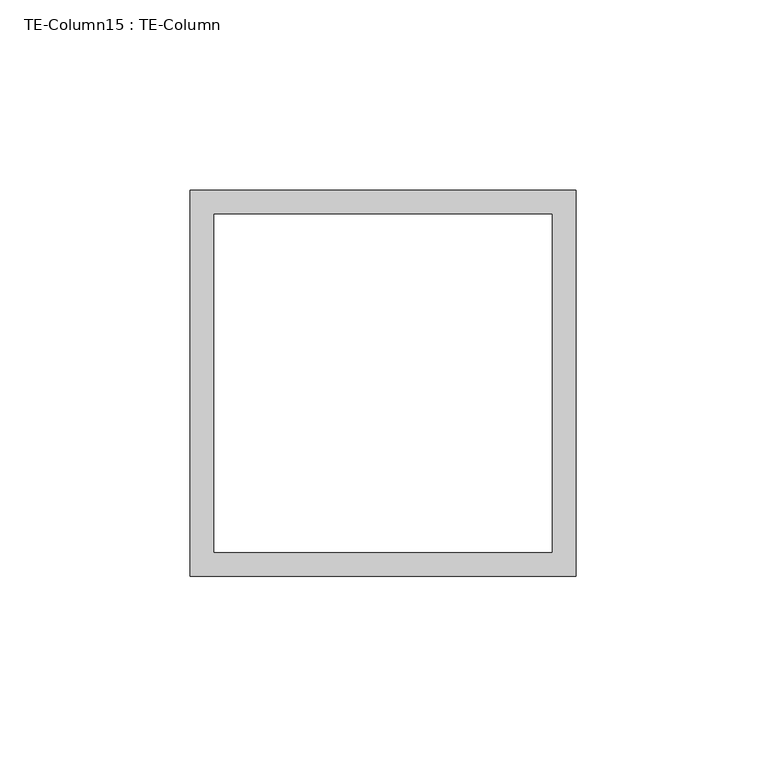
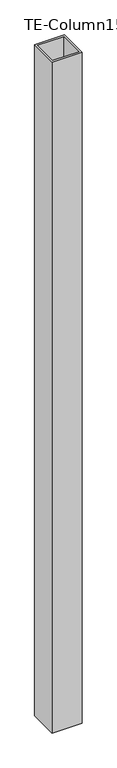
"""IFC4 building model written with IfcOpenShell, lengths in millimetres: proxy geometry, TE-Column15 : TE-Column."""

from ifc_helpers import new_model, si_unit, frame, origin, place, context, project, spatial, polyline, outline, extrude, source, transform, mapped, element, save


def te_column15_te_column_72f26b47(model_context):
    return source(origin(), model_context, "Body", "SweptSolid", [
        extrude(outline(polyline([(590318.6434739, -534093.4913841), (590217.0434739, -534093.4913841), (590217.0434739, -533991.8913841), (590318.6434739, -533991.8913841), (590318.6434739, -534093.4913841)]), holes=[polyline([(590312.2934739, -533998.2413841), (590223.3934739, -533998.2413841), (590223.3934739, -534087.1413841), (590312.2934739, -534087.1413841), (590312.2934739, -533998.2413841)])]), frame((0.0, 0.0, 28.575), z_axis=(0.0, 0.0, 1.0), x_axis=(1.0, 0.0, 0.0)), (0.0, 0.0, 1.0), 2406.65),
    ])


if __name__ == "__main__":
    model = new_model("IFC4")
    model_context = context("Model", 3, world=origin())
    ifc_project = project(units=[si_unit("LENGTHUNIT", "METRE", prefix="MILLI")], contexts=[model_context])
    site = spatial("IfcSite", under=ifc_project)
    building = spatial("IfcBuilding", under=site)
    placement = place(None, origin())
    te_column15_te_column_shape = te_column15_te_column_72f26b47(model_context)
    element("IfcBuildingElementProxy", 1, Name="TE-Column15 : TE-Column", ObjectType="TE-Column15 : TE-Column", at=placement, inside=building, context=model_context, shape_type="MappedRepresentation", body=[
        mapped(te_column15_te_column_shape, transform((0.0, 0.0, 0.0), x_axis=(1.0, 0.0, 0.0), y_axis=(0.0, 1.0, 0.0), z_axis=(0.0, 0.0, 1.0))),
    ])
    save(model, "model.ifc")

# Revit data of these elements
# Element 1 (IfcBuildingElementProxy, "TE-Column15 : TE-Column")
#   Materials on its faces: "4\"X4\" GALV. HSS TUBING"
# Materials
#   "4\"X4\" GALV. HSS TUBING": class "Generic", colour RGB 211 211 207, transparency 0, Cost = 0
